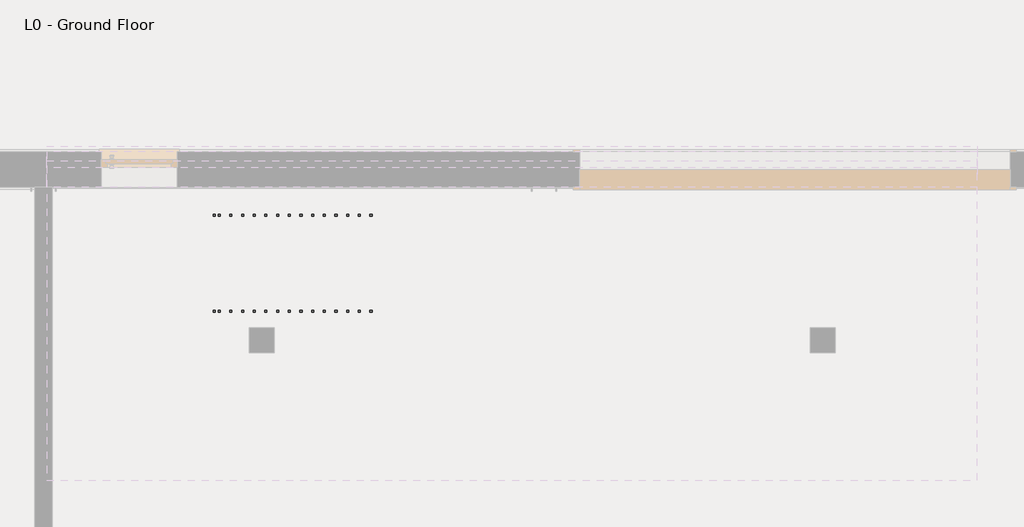
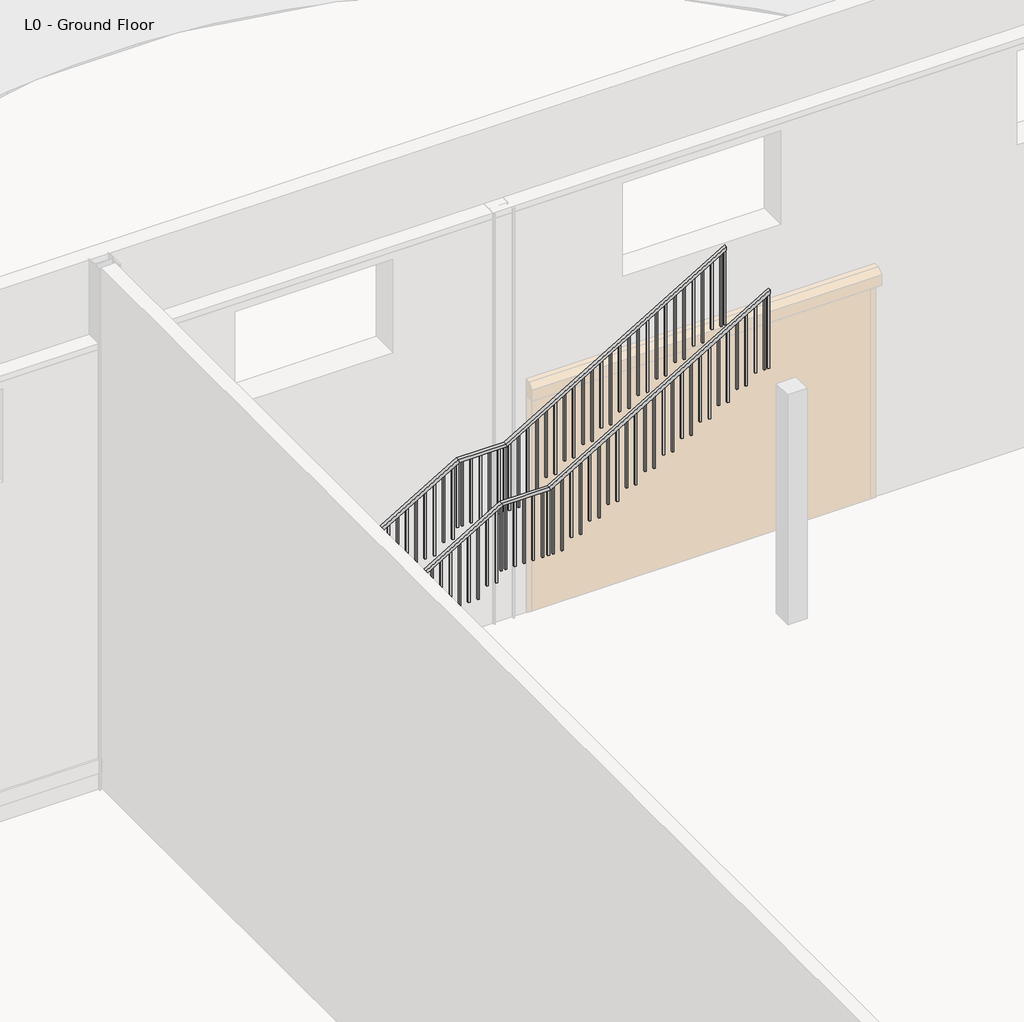
# One storey, part 12 of 14: 2 railings.
"""IFC4 building model written with IfcOpenShell, lengths in millimetres."""

from ifc_helpers import new_model, si_unit, frame, origin, place, context, project, spatial, polyline, outline, extrude, faceted_brep, element, save

model = new_model("IFC4")

# Units and contexts
model_context = context("Model", 3, world=origin())
ifc_project = project(units=[si_unit("LENGTHUNIT", "METRE", prefix="MILLI")], contexts=[model_context])

# Site, building, storey
site = spatial("IfcSite", under=ifc_project)
building = spatial("IfcBuilding", under=site)
storey = spatial("IfcBuildingStorey", under=building, Name="L0 - Ground Floor", Elevation=0.0)

# Railings
placement = place(None, origin())
element("IfcRailing", 1, ObjectType="1100mm", at=placement, inside=storey, context=model_context, shape_type="SolidModel", body=[
    faceted_brep([(12896.9831159, 5374.1380918, 1266.6666667), (12896.9831159, 5374.1380918, 1208.4792885), (12896.9831159, 5324.1380918, 1208.4792885), (12896.9831159, 5324.1380918, 1266.6666667), (15976.9831159, 5374.1380918, 3100.0), (15990.7379111, 5374.1380918, 3050.0), (15990.7379111, 5324.1380918, 3050.0), (15976.9831159, 5324.1380918, 3100.0), (16696.9831159, 5374.1380918, 3100.0), (16710.7379111, 5374.1380918, 3050.0), (16710.7379111, 5324.1380918, 3050.0), (16696.9831159, 5324.1380918, 3100.0), (20056.9831159, 5374.1380918, 5100.0), (20056.9831159, 5324.1380918, 5100.0), (20056.9831159, 5324.1380918, 5041.8126219), (20056.9831159, 5374.1380918, 5041.8126219)], [[[0, 1, 2, 3]], [[1, 0, 4, 5]], [[2, 1, 5, 6]], [[3, 2, 6, 7]], [[0, 3, 7, 4]], [[5, 4, 8, 9]], [[6, 5, 9, 10]], [[7, 6, 10, 11]], [[4, 7, 11, 8]], [[12, 13, 14, 15]], [[9, 8, 12, 15]], [[10, 9, 15, 14]], [[11, 10, 14, 13]], [[8, 11, 13, 12]]]),
    extrude(outline(polyline([(4992.705479, 19974.4831159), (3833.3333333, 19974.4831159), (3833.3333333, 19999.4831159), (5007.5864314, 19999.4831159), (4992.705479, 19974.4831159)])), frame((0.0, 5336.6380918, 0.0), z_axis=(0.0, 1.0, 0.0), x_axis=(0.0, 0.0, 1.0)), (0.0, 0.0, 1.0), 25.0),
    extrude(outline(polyline([(4909.3721457, 19834.4831159), (3833.3333333, 19834.4831159), (3833.3333333, 19859.4831159), (4924.253098, 19859.4831159), (4909.3721457, 19834.4831159)])), frame((0.0, 5336.6380918, 0.0), z_axis=(0.0, 1.0, 0.0), x_axis=(0.0, 0.0, 1.0)), (0.0, 0.0, 1.0), 25.0),
    extrude(outline(polyline([(4826.0388123, 19694.4831159), (3666.6666667, 19694.4831159), (3666.6666667, 19719.4831159), (4840.9197647, 19719.4831159), (4826.0388123, 19694.4831159)])), frame((0.0, 5336.6380918, 0.0), z_axis=(0.0, 1.0, 0.0), x_axis=(0.0, 0.0, 1.0)), (0.0, 0.0, 1.0), 25.0),
    extrude(outline(polyline([(4742.705479, 19554.4831159), (3666.6666667, 19554.4831159), (3666.6666667, 19579.4831159), (4757.5864314, 19579.4831159), (4742.705479, 19554.4831159)])), frame((0.0, 5336.6380918, 0.0), z_axis=(0.0, 1.0, 0.0), x_axis=(0.0, 0.0, 1.0)), (0.0, 0.0, 1.0), 25.0),
    extrude(outline(polyline([(4659.3721457, 19414.4831159), (3500.0, 19414.4831159), (3500.0, 19439.4831159), (4674.253098, 19439.4831159), (4659.3721457, 19414.4831159)])), frame((0.0, 5336.6380918, 0.0), z_axis=(0.0, 1.0, 0.0), x_axis=(0.0, 0.0, 1.0)), (0.0, 0.0, 1.0), 25.0),
    extrude(outline(polyline([(4576.0388123, 19274.4831159), (3500.0, 19274.4831159), (3500.0, 19299.4831159), (4590.9197647, 19299.4831159), (4576.0388123, 19274.4831159)])), frame((0.0, 5336.6380918, 0.0), z_axis=(0.0, 1.0, 0.0), x_axis=(0.0, 0.0, 1.0)), (0.0, 0.0, 1.0), 25.0),
    extrude(outline(polyline([(4492.705479, 19134.4831159), (3333.3333333, 19134.4831159), (3333.3333333, 19159.4831159), (4507.5864314, 19159.4831159), (4492.705479, 19134.4831159)])), frame((0.0, 5336.6380918, 0.0), z_axis=(0.0, 1.0, 0.0), x_axis=(0.0, 0.0, 1.0)), (0.0, 0.0, 1.0), 25.0),
    extrude(outline(polyline([(4409.3721457, 18994.4831159), (3333.3333333, 18994.4831159), (3333.3333333, 19019.4831159), (4424.253098, 19019.4831159), (4409.3721457, 18994.4831159)])), frame((0.0, 5336.6380918, 0.0), z_axis=(0.0, 1.0, 0.0), x_axis=(0.0, 0.0, 1.0)), (0.0, 0.0, 1.0), 25.0),
    extrude(outline(polyline([(4326.0388123, 18854.4831159), (3166.6666667, 18854.4831159), (3166.6666667, 18879.4831159), (4340.9197647, 18879.4831159), (4326.0388123, 18854.4831159)])), frame((0.0, 5336.6380918, 0.0), z_axis=(0.0, 1.0, 0.0), x_axis=(0.0, 0.0, 1.0)), (0.0, 0.0, 1.0), 25.0),
    extrude(outline(polyline([(4242.705479, 18714.4831159), (3166.6666667, 18714.4831159), (3166.6666667, 18739.4831159), (4257.5864314, 18739.4831159), (4242.705479, 18714.4831159)])), frame((0.0, 5336.6380918, 0.0), z_axis=(0.0, 1.0, 0.0), x_axis=(0.0, 0.0, 1.0)), (0.0, 0.0, 1.0), 25.0),
    extrude(outline(polyline([(4159.3721457, 18574.4831159), (3000.0, 18574.4831159), (3000.0, 18599.4831159), (4174.253098, 18599.4831159), (4159.3721457, 18574.4831159)])), frame((0.0, 5336.6380918, 0.0), z_axis=(0.0, 1.0, 0.0), x_axis=(0.0, 0.0, 1.0)), (0.0, 0.0, 1.0), 25.0),
    extrude(outline(polyline([(4076.0388123, 18434.4831159), (3000.0, 18434.4831159), (3000.0, 18459.4831159), (4090.9197647, 18459.4831159), (4076.0388123, 18434.4831159)])), frame((0.0, 5336.6380918, 0.0), z_axis=(0.0, 1.0, 0.0), x_axis=(0.0, 0.0, 1.0)), (0.0, 0.0, 1.0), 25.0),
    extrude(outline(polyline([(3992.705479, 18294.4831159), (2833.3333333, 18294.4831159), (2833.3333333, 18319.4831159), (4007.5864314, 18319.4831159), (3992.705479, 18294.4831159)])), frame((0.0, 5336.6380918, 0.0), z_axis=(0.0, 1.0, 0.0), x_axis=(0.0, 0.0, 1.0)), (0.0, 0.0, 1.0), 25.0),
    extrude(outline(polyline([(3909.3721457, 18154.4831159), (2833.3333333, 18154.4831159), (2833.3333333, 18179.4831159), (3924.253098, 18179.4831159), (3909.3721457, 18154.4831159)])), frame((0.0, 5336.6380918, 0.0), z_axis=(0.0, 1.0, 0.0), x_axis=(0.0, 0.0, 1.0)), (0.0, 0.0, 1.0), 25.0),
    extrude(outline(polyline([(3826.0388123, 18014.4831159), (2666.6666667, 18014.4831159), (2666.6666667, 18039.4831159), (3840.9197647, 18039.4831159), (3826.0388123, 18014.4831159)])), frame((0.0, 5336.6380918, 0.0), z_axis=(0.0, 1.0, 0.0), x_axis=(0.0, 0.0, 1.0)), (0.0, 0.0, 1.0), 25.0),
    extrude(outline(polyline([(3742.705479, 17874.4831159), (2666.6666667, 17874.4831159), (2666.6666667, 17899.4831159), (3757.5864314, 17899.4831159), (3742.705479, 17874.4831159)])), frame((0.0, 5336.6380918, 0.0), z_axis=(0.0, 1.0, 0.0), x_axis=(0.0, 0.0, 1.0)), (0.0, 0.0, 1.0), 25.0),
    extrude(outline(polyline([(3659.3721457, 17734.4831159), (2500.0, 17734.4831159), (2500.0, 17759.4831159), (3674.253098, 17759.4831159), (3659.3721457, 17734.4831159)])), frame((0.0, 5336.6380918, 0.0), z_axis=(0.0, 1.0, 0.0), x_axis=(0.0, 0.0, 1.0)), (0.0, 0.0, 1.0), 25.0),
    extrude(outline(polyline([(3576.0388123, 17594.4831159), (2500.0, 17594.4831159), (2500.0, 17619.4831159), (3590.9197647, 17619.4831159), (3576.0388123, 17594.4831159)])), frame((0.0, 5336.6380918, 0.0), z_axis=(0.0, 1.0, 0.0), x_axis=(0.0, 0.0, 1.0)), (0.0, 0.0, 1.0), 25.0),
    extrude(outline(polyline([(3492.705479, 17454.4831159), (2333.3333333, 17454.4831159), (2333.3333333, 17479.4831159), (3507.5864314, 17479.4831159), (3492.705479, 17454.4831159)])), frame((0.0, 5336.6380918, 0.0), z_axis=(0.0, 1.0, 0.0), x_axis=(0.0, 0.0, 1.0)), (0.0, 0.0, 1.0), 25.0),
    extrude(outline(polyline([(3409.3721457, 17314.4831159), (2333.3333333, 17314.4831159), (2333.3333333, 17339.4831159), (3424.253098, 17339.4831159), (3409.3721457, 17314.4831159)])), frame((0.0, 5336.6380918, 0.0), z_axis=(0.0, 1.0, 0.0), x_axis=(0.0, 0.0, 1.0)), (0.0, 0.0, 1.0), 25.0),
    extrude(outline(polyline([(3326.0388123, 17174.4831159), (2166.6666667, 17174.4831159), (2166.6666667, 17199.4831159), (3340.9197647, 17199.4831159), (3326.0388123, 17174.4831159)])), frame((0.0, 5336.6380918, 0.0), z_axis=(0.0, 1.0, 0.0), x_axis=(0.0, 0.0, 1.0)), (0.0, 0.0, 1.0), 25.0),
    extrude(outline(polyline([(3242.705479, 17034.4831159), (2166.6666667, 17034.4831159), (2166.6666667, 17059.4831159), (3257.5864314, 17059.4831159), (3242.705479, 17034.4831159)])), frame((0.0, 5336.6380918, 0.0), z_axis=(0.0, 1.0, 0.0), x_axis=(0.0, 0.0, 1.0)), (0.0, 0.0, 1.0), 25.0),
    extrude(outline(polyline([(3159.3721457, 16894.4831159), (2000.0, 16894.4831159), (2000.0, 16919.4831159), (3174.253098, 16919.4831159), (3159.3721457, 16894.4831159)])), frame((0.0, 5336.6380918, 0.0), z_axis=(0.0, 1.0, 0.0), x_axis=(0.0, 0.0, 1.0)), (0.0, 0.0, 1.0), 25.0),
    extrude(outline(polyline([(3076.0388123, 16754.4831159), (2000.0, 16754.4831159), (2000.0, 16779.4831159), (3090.9197647, 16779.4831159), (3076.0388123, 16754.4831159)])), frame((0.0, 5336.6380918, 0.0), z_axis=(0.0, 1.0, 0.0), x_axis=(0.0, 0.0, 1.0)), (0.0, 0.0, 1.0), 25.0),
    extrude(outline(polyline([(16594.4831159, 5336.6380918), (16594.4831159, 5361.6380918), (16619.4831159, 5361.6380918), (16619.4831159, 5336.6380918), (16594.4831159, 5336.6380918)])), frame((0.0, 0.0, 2000.0), z_axis=(0.0, 0.0, 1.0), x_axis=(1.0, 0.0, 0.0)), (0.0, 0.0, 1.0), 1050.0),
    extrude(outline(polyline([(16454.4831159, 5336.6380918), (16454.4831159, 5361.6380918), (16479.4831159, 5361.6380918), (16479.4831159, 5336.6380918), (16454.4831159, 5336.6380918)])), frame((0.0, 0.0, 2000.0), z_axis=(0.0, 0.0, 1.0), x_axis=(1.0, 0.0, 0.0)), (0.0, 0.0, 1.0), 1050.0),
    extrude(outline(polyline([(16314.4831159, 5336.6380918), (16314.4831159, 5361.6380918), (16339.4831159, 5361.6380918), (16339.4831159, 5336.6380918), (16314.4831159, 5336.6380918)])), frame((0.0, 0.0, 2000.0), z_axis=(0.0, 0.0, 1.0), x_axis=(1.0, 0.0, 0.0)), (0.0, 0.0, 1.0), 1050.0),
    extrude(outline(polyline([(16174.4831159, 5336.6380918), (16174.4831159, 5361.6380918), (16199.4831159, 5361.6380918), (16199.4831159, 5336.6380918), (16174.4831159, 5336.6380918)])), frame((0.0, 0.0, 2000.0), z_axis=(0.0, 0.0, 1.0), x_axis=(1.0, 0.0, 0.0)), (0.0, 0.0, 1.0), 1050.0),
    extrude(outline(polyline([(16034.4831159, 5336.6380918), (16034.4831159, 5361.6380918), (16059.4831159, 5361.6380918), (16059.4831159, 5336.6380918), (16034.4831159, 5336.6380918)])), frame((0.0, 0.0, 2000.0), z_axis=(0.0, 0.0, 1.0), x_axis=(1.0, 0.0, 0.0)), (0.0, 0.0, 1.0), 1050.0),
    extrude(outline(polyline([(2992.705479, 15894.4831159), (1833.3333333, 15894.4831159), (1833.3333333, 15919.4831159), (3007.5864314, 15919.4831159), (2992.705479, 15894.4831159)])), frame((0.0, 5336.6380918, 0.0), z_axis=(0.0, 1.0, 0.0), x_axis=(0.0, 0.0, 1.0)), (0.0, 0.0, 1.0), 25.0),
    extrude(outline(polyline([(2909.3721457, 15754.4831159), (1833.3333333, 15754.4831159), (1833.3333333, 15779.4831159), (2924.253098, 15779.4831159), (2909.3721457, 15754.4831159)])), frame((0.0, 5336.6380918, 0.0), z_axis=(0.0, 1.0, 0.0), x_axis=(0.0, 0.0, 1.0)), (0.0, 0.0, 1.0), 25.0),
    extrude(outline(polyline([(2826.0388123, 15614.4831159), (1666.6666667, 15614.4831159), (1666.6666667, 15639.4831159), (2840.9197647, 15639.4831159), (2826.0388123, 15614.4831159)])), frame((0.0, 5336.6380918, 0.0), z_axis=(0.0, 1.0, 0.0), x_axis=(0.0, 0.0, 1.0)), (0.0, 0.0, 1.0), 25.0),
    extrude(outline(polyline([(2742.705479, 15474.4831159), (1666.6666667, 15474.4831159), (1666.6666667, 15499.4831159), (2757.5864314, 15499.4831159), (2742.705479, 15474.4831159)])), frame((0.0, 5336.6380918, 0.0), z_axis=(0.0, 1.0, 0.0), x_axis=(0.0, 0.0, 1.0)), (0.0, 0.0, 1.0), 25.0),
    extrude(outline(polyline([(2659.3721457, 15334.4831159), (1500.0, 15334.4831159), (1500.0, 15359.4831159), (2674.253098, 15359.4831159), (2659.3721457, 15334.4831159)])), frame((0.0, 5336.6380918, 0.0), z_axis=(0.0, 1.0, 0.0), x_axis=(0.0, 0.0, 1.0)), (0.0, 0.0, 1.0), 25.0),
    extrude(outline(polyline([(2576.0388123, 15194.4831159), (1500.0, 15194.4831159), (1500.0, 15219.4831159), (2590.9197647, 15219.4831159), (2576.0388123, 15194.4831159)])), frame((0.0, 5336.6380918, 0.0), z_axis=(0.0, 1.0, 0.0), x_axis=(0.0, 0.0, 1.0)), (0.0, 0.0, 1.0), 25.0),
    extrude(outline(polyline([(2492.705479, 15054.4831159), (1333.3333333, 15054.4831159), (1333.3333333, 15079.4831159), (2507.5864314, 15079.4831159), (2492.705479, 15054.4831159)])), frame((0.0, 5336.6380918, 0.0), z_axis=(0.0, 1.0, 0.0), x_axis=(0.0, 0.0, 1.0)), (0.0, 0.0, 1.0), 25.0),
    extrude(outline(polyline([(2409.3721457, 14914.4831159), (1333.3333333, 14914.4831159), (1333.3333333, 14939.4831159), (2424.253098, 14939.4831159), (2409.3721457, 14914.4831159)])), frame((0.0, 5336.6380918, 0.0), z_axis=(0.0, 1.0, 0.0), x_axis=(0.0, 0.0, 1.0)), (0.0, 0.0, 1.0), 25.0),
    extrude(outline(polyline([(2326.0388123, 14774.4831159), (1166.6666667, 14774.4831159), (1166.6666667, 14799.4831159), (2340.9197647, 14799.4831159), (2326.0388123, 14774.4831159)])), frame((0.0, 5336.6380918, 0.0), z_axis=(0.0, 1.0, 0.0), x_axis=(0.0, 0.0, 1.0)), (0.0, 0.0, 1.0), 25.0),
    extrude(outline(polyline([(2242.705479, 14634.4831159), (1166.6666667, 14634.4831159), (1166.6666667, 14659.4831159), (2257.5864314, 14659.4831159), (2242.705479, 14634.4831159)])), frame((0.0, 5336.6380918, 0.0), z_axis=(0.0, 1.0, 0.0), x_axis=(0.0, 0.0, 1.0)), (0.0, 0.0, 1.0), 25.0),
    extrude(outline(polyline([(2159.3721457, 14494.4831159), (1000.0, 14494.4831159), (1000.0, 14519.4831159), (2174.253098, 14519.4831159), (2159.3721457, 14494.4831159)])), frame((0.0, 5336.6380918, 0.0), z_axis=(0.0, 1.0, 0.0), x_axis=(0.0, 0.0, 1.0)), (0.0, 0.0, 1.0), 25.0),
    extrude(outline(polyline([(2076.0388123, 14354.4831159), (1000.0, 14354.4831159), (1000.0, 14379.4831159), (2090.9197647, 14379.4831159), (2076.0388123, 14354.4831159)])), frame((0.0, 5336.6380918, 0.0), z_axis=(0.0, 1.0, 0.0), x_axis=(0.0, 0.0, 1.0)), (0.0, 0.0, 1.0), 25.0),
    extrude(outline(polyline([(1992.705479, 14214.4831159), (833.3333333, 14214.4831159), (833.3333333, 14239.4831159), (2007.5864314, 14239.4831159), (1992.705479, 14214.4831159)])), frame((0.0, 5336.6380918, 0.0), z_axis=(0.0, 1.0, 0.0), x_axis=(0.0, 0.0, 1.0)), (0.0, 0.0, 1.0), 25.0),
    extrude(outline(polyline([(1909.3721457, 14074.4831159), (833.3333333, 14074.4831159), (833.3333333, 14099.4831159), (1924.253098, 14099.4831159), (1909.3721457, 14074.4831159)])), frame((0.0, 5336.6380918, 0.0), z_axis=(0.0, 1.0, 0.0), x_axis=(0.0, 0.0, 1.0)), (0.0, 0.0, 1.0), 25.0),
    extrude(outline(polyline([(1826.0388123, 13934.4831159), (666.6666667, 13934.4831159), (666.6666667, 13959.4831159), (1840.9197647, 13959.4831159), (1826.0388123, 13934.4831159)])), frame((0.0, 5336.6380918, 0.0), z_axis=(0.0, 1.0, 0.0), x_axis=(0.0, 0.0, 1.0)), (0.0, 0.0, 1.0), 25.0),
    extrude(outline(polyline([(1742.705479, 13794.4831159), (666.6666667, 13794.4831159), (666.6666667, 13819.4831159), (1757.5864314, 13819.4831159), (1742.705479, 13794.4831159)])), frame((0.0, 5336.6380918, 0.0), z_axis=(0.0, 1.0, 0.0), x_axis=(0.0, 0.0, 1.0)), (0.0, 0.0, 1.0), 25.0),
    extrude(outline(polyline([(1659.3721457, 13654.4831159), (500.0, 13654.4831159), (500.0, 13679.4831159), (1674.253098, 13679.4831159), (1659.3721457, 13654.4831159)])), frame((0.0, 5336.6380918, 0.0), z_axis=(0.0, 1.0, 0.0), x_axis=(0.0, 0.0, 1.0)), (0.0, 0.0, 1.0), 25.0),
    extrude(outline(polyline([(1576.0388123, 13514.4831159), (500.0, 13514.4831159), (500.0, 13539.4831159), (1590.9197647, 13539.4831159), (1576.0388123, 13514.4831159)])), frame((0.0, 5336.6380918, 0.0), z_axis=(0.0, 1.0, 0.0), x_axis=(0.0, 0.0, 1.0)), (0.0, 0.0, 1.0), 25.0),
    extrude(outline(polyline([(1492.705479, 13374.4831159), (333.3333333, 13374.4831159), (333.3333333, 13399.4831159), (1507.5864314, 13399.4831159), (1492.705479, 13374.4831159)])), frame((0.0, 5336.6380918, 0.0), z_axis=(0.0, 1.0, 0.0), x_axis=(0.0, 0.0, 1.0)), (0.0, 0.0, 1.0), 25.0),
    extrude(outline(polyline([(1409.3721457, 13234.4831159), (333.3333333, 13234.4831159), (333.3333333, 13259.4831159), (1424.253098, 13259.4831159), (1409.3721457, 13234.4831159)])), frame((0.0, 5336.6380918, 0.0), z_axis=(0.0, 1.0, 0.0), x_axis=(0.0, 0.0, 1.0)), (0.0, 0.0, 1.0), 25.0),
    extrude(outline(polyline([(1326.0388123, 13094.4831159), (166.6666667, 13094.4831159), (166.6666667, 13119.4831159), (1340.9197647, 13119.4831159), (1326.0388123, 13094.4831159)])), frame((0.0, 5336.6380918, 0.0), z_axis=(0.0, 1.0, 0.0), x_axis=(0.0, 0.0, 1.0)), (0.0, 0.0, 1.0), 25.0),
    extrude(outline(polyline([(1242.705479, 12954.4831159), (166.6666667, 12954.4831159), (166.6666667, 12979.4831159), (1257.5864314, 12979.4831159), (1242.705479, 12954.4831159)])), frame((0.0, 5336.6380918, 0.0), z_axis=(0.0, 1.0, 0.0), x_axis=(0.0, 0.0, 1.0)), (0.0, 0.0, 1.0), 25.0),
    extrude(outline(polyline([(16684.4831159, 5336.6380918), (16684.4831159, 5361.6380918), (16709.4831159, 5361.6380918), (16709.4831159, 5336.6380918), (16684.4831159, 5336.6380918)])), frame((0.0, 0.0, 2000.0), z_axis=(0.0, 0.0, 1.0), x_axis=(1.0, 0.0, 0.0)), (0.0, 0.0, 1.0), 1050.0),
    extrude(outline(polyline([(15964.4831159, 5336.6380918), (15964.4831159, 5361.6380918), (15989.4831159, 5361.6380918), (15989.4831159, 5336.6380918), (15964.4831159, 5336.6380918)])), frame((0.0, 0.0, 2000.0), z_axis=(0.0, 0.0, 1.0), x_axis=(1.0, 0.0, 0.0)), (0.0, 0.0, 1.0), 1050.0),
    extrude(outline(polyline([(5026.9316695, 20031.9831159), (3833.3333333, 20031.9831159), (3833.3333333, 20056.9831159), (5041.8126219, 20056.9831159), (5026.9316695, 20031.9831159)])), frame((0.0, 5336.6380918, 0.0), z_axis=(0.0, 1.0, 0.0), x_axis=(0.0, 0.0, 1.0)), (0.0, 0.0, 1.0), 25.0),
    extrude(outline(polyline([(1208.4792885, 12896.9831159), (166.6666667, 12896.9831159), (166.6666667, 12921.9831159), (1223.3602409, 12921.9831159), (1208.4792885, 12896.9831159)])), frame((0.0, 5336.6380918, 0.0), z_axis=(0.0, 1.0, 0.0), x_axis=(0.0, 0.0, 1.0)), (0.0, 0.0, 1.0), 25.0),
])
element("IfcRailing", 2, ObjectType="1100mm", at=placement, inside=storey, context=model_context, shape_type="SolidModel", body=[
    faceted_brep([(12896.9831159, 6523.3380918, 1266.6666667), (12896.9831159, 6523.3380918, 1208.4792885), (12896.9831159, 6473.3380918, 1208.4792885), (12896.9831159, 6473.3380918, 1266.6666667), (15976.9831159, 6523.3380918, 3100.0), (15990.7379111, 6523.3380918, 3050.0), (15990.7379111, 6473.3380918, 3050.0), (15976.9831159, 6473.3380918, 3100.0), (16696.9831159, 6523.3380918, 3100.0), (16710.7379111, 6523.3380918, 3050.0), (16710.7379111, 6473.3380918, 3050.0), (16696.9831159, 6473.3380918, 3100.0), (20056.9831159, 6523.3380918, 5100.0), (20056.9831159, 6473.3380918, 5100.0), (20056.9831159, 6473.3380918, 5041.8126219), (20056.9831159, 6523.3380918, 5041.8126219)], [[[0, 1, 2, 3]], [[1, 0, 4, 5]], [[2, 1, 5, 6]], [[3, 2, 6, 7]], [[0, 3, 7, 4]], [[5, 4, 8, 9]], [[6, 5, 9, 10]], [[7, 6, 10, 11]], [[4, 7, 11, 8]], [[12, 13, 14, 15]], [[9, 8, 12, 15]], [[10, 9, 15, 14]], [[11, 10, 14, 13]], [[8, 11, 13, 12]]]),
    extrude(outline(polyline([(3833.3333333, 19974.4831159), (3833.3333333, 19999.4831159), (5007.5864314, 19999.4831159), (4992.705479, 19974.4831159), (3833.3333333, 19974.4831159)])), frame((0.0, 6485.8380918, 0.0), z_axis=(0.0, 1.0, 0.0), x_axis=(0.0, 0.0, 1.0)), (0.0, 0.0, 1.0), 25.0),
    extrude(outline(polyline([(3833.3333333, 19834.4831159), (3833.3333333, 19859.4831159), (4924.253098, 19859.4831159), (4909.3721457, 19834.4831159), (3833.3333333, 19834.4831159)])), frame((0.0, 6485.8380918, 0.0), z_axis=(0.0, 1.0, 0.0), x_axis=(0.0, 0.0, 1.0)), (0.0, 0.0, 1.0), 25.0),
    extrude(outline(polyline([(3666.6666667, 19694.4831159), (3666.6666667, 19719.4831159), (4840.9197647, 19719.4831159), (4826.0388123, 19694.4831159), (3666.6666667, 19694.4831159)])), frame((0.0, 6485.8380918, 0.0), z_axis=(0.0, 1.0, 0.0), x_axis=(0.0, 0.0, 1.0)), (0.0, 0.0, 1.0), 25.0),
    extrude(outline(polyline([(3666.6666667, 19554.4831159), (3666.6666667, 19579.4831159), (4757.5864314, 19579.4831159), (4742.705479, 19554.4831159), (3666.6666667, 19554.4831159)])), frame((0.0, 6485.8380918, 0.0), z_axis=(0.0, 1.0, 0.0), x_axis=(0.0, 0.0, 1.0)), (0.0, 0.0, 1.0), 25.0),
    extrude(outline(polyline([(3500.0, 19414.4831159), (3500.0, 19439.4831159), (4674.253098, 19439.4831159), (4659.3721457, 19414.4831159), (3500.0, 19414.4831159)])), frame((0.0, 6485.8380918, 0.0), z_axis=(0.0, 1.0, 0.0), x_axis=(0.0, 0.0, 1.0)), (0.0, 0.0, 1.0), 25.0),
    extrude(outline(polyline([(3500.0, 19274.4831159), (3500.0, 19299.4831159), (4590.9197647, 19299.4831159), (4576.0388123, 19274.4831159), (3500.0, 19274.4831159)])), frame((0.0, 6485.8380918, 0.0), z_axis=(0.0, 1.0, 0.0), x_axis=(0.0, 0.0, 1.0)), (0.0, 0.0, 1.0), 25.0),
    extrude(outline(polyline([(3333.3333333, 19134.4831159), (3333.3333333, 19159.4831159), (4507.5864314, 19159.4831159), (4492.705479, 19134.4831159), (3333.3333333, 19134.4831159)])), frame((0.0, 6485.8380918, 0.0), z_axis=(0.0, 1.0, 0.0), x_axis=(0.0, 0.0, 1.0)), (0.0, 0.0, 1.0), 25.0),
    extrude(outline(polyline([(3333.3333333, 18994.4831159), (3333.3333333, 19019.4831159), (4424.253098, 19019.4831159), (4409.3721457, 18994.4831159), (3333.3333333, 18994.4831159)])), frame((0.0, 6485.8380918, 0.0), z_axis=(0.0, 1.0, 0.0), x_axis=(0.0, 0.0, 1.0)), (0.0, 0.0, 1.0), 25.0),
    extrude(outline(polyline([(3166.6666667, 18854.4831159), (3166.6666667, 18879.4831159), (4340.9197647, 18879.4831159), (4326.0388123, 18854.4831159), (3166.6666667, 18854.4831159)])), frame((0.0, 6485.8380918, 0.0), z_axis=(0.0, 1.0, 0.0), x_axis=(0.0, 0.0, 1.0)), (0.0, 0.0, 1.0), 25.0),
    extrude(outline(polyline([(3166.6666667, 18714.4831159), (3166.6666667, 18739.4831159), (4257.5864314, 18739.4831159), (4242.705479, 18714.4831159), (3166.6666667, 18714.4831159)])), frame((0.0, 6485.8380918, 0.0), z_axis=(0.0, 1.0, 0.0), x_axis=(0.0, 0.0, 1.0)), (0.0, 0.0, 1.0), 25.0),
    extrude(outline(polyline([(3000.0, 18574.4831159), (3000.0, 18599.4831159), (4174.253098, 18599.4831159), (4159.3721457, 18574.4831159), (3000.0, 18574.4831159)])), frame((0.0, 6485.8380918, 0.0), z_axis=(0.0, 1.0, 0.0), x_axis=(0.0, 0.0, 1.0)), (0.0, 0.0, 1.0), 25.0),
    extrude(outline(polyline([(3000.0, 18434.4831159), (3000.0, 18459.4831159), (4090.9197647, 18459.4831159), (4076.0388123, 18434.4831159), (3000.0, 18434.4831159)])), frame((0.0, 6485.8380918, 0.0), z_axis=(0.0, 1.0, 0.0), x_axis=(0.0, 0.0, 1.0)), (0.0, 0.0, 1.0), 25.0),
    extrude(outline(polyline([(2833.3333333, 18294.4831159), (2833.3333333, 18319.4831159), (4007.5864314, 18319.4831159), (3992.705479, 18294.4831159), (2833.3333333, 18294.4831159)])), frame((0.0, 6485.8380918, 0.0), z_axis=(0.0, 1.0, 0.0), x_axis=(0.0, 0.0, 1.0)), (0.0, 0.0, 1.0), 25.0),
    extrude(outline(polyline([(2833.3333333, 18154.4831159), (2833.3333333, 18179.4831159), (3924.253098, 18179.4831159), (3909.3721457, 18154.4831159), (2833.3333333, 18154.4831159)])), frame((0.0, 6485.8380918, 0.0), z_axis=(0.0, 1.0, 0.0), x_axis=(0.0, 0.0, 1.0)), (0.0, 0.0, 1.0), 25.0),
    extrude(outline(polyline([(2666.6666667, 18014.4831159), (2666.6666667, 18039.4831159), (3840.9197647, 18039.4831159), (3826.0388123, 18014.4831159), (2666.6666667, 18014.4831159)])), frame((0.0, 6485.8380918, 0.0), z_axis=(0.0, 1.0, 0.0), x_axis=(0.0, 0.0, 1.0)), (0.0, 0.0, 1.0), 25.0),
    extrude(outline(polyline([(2666.6666667, 17874.4831159), (2666.6666667, 17899.4831159), (3757.5864314, 17899.4831159), (3742.705479, 17874.4831159), (2666.6666667, 17874.4831159)])), frame((0.0, 6485.8380918, 0.0), z_axis=(0.0, 1.0, 0.0), x_axis=(0.0, 0.0, 1.0)), (0.0, 0.0, 1.0), 25.0),
    extrude(outline(polyline([(2500.0, 17734.4831159), (2500.0, 17759.4831159), (3674.253098, 17759.4831159), (3659.3721457, 17734.4831159), (2500.0, 17734.4831159)])), frame((0.0, 6485.8380918, 0.0), z_axis=(0.0, 1.0, 0.0), x_axis=(0.0, 0.0, 1.0)), (0.0, 0.0, 1.0), 25.0),
    extrude(outline(polyline([(2500.0, 17594.4831159), (2500.0, 17619.4831159), (3590.9197647, 17619.4831159), (3576.0388123, 17594.4831159), (2500.0, 17594.4831159)])), frame((0.0, 6485.8380918, 0.0), z_axis=(0.0, 1.0, 0.0), x_axis=(0.0, 0.0, 1.0)), (0.0, 0.0, 1.0), 25.0),
    extrude(outline(polyline([(2333.3333333, 17454.4831159), (2333.3333333, 17479.4831159), (3507.5864314, 17479.4831159), (3492.705479, 17454.4831159), (2333.3333333, 17454.4831159)])), frame((0.0, 6485.8380918, 0.0), z_axis=(0.0, 1.0, 0.0), x_axis=(0.0, 0.0, 1.0)), (0.0, 0.0, 1.0), 25.0),
    extrude(outline(polyline([(2333.3333333, 17314.4831159), (2333.3333333, 17339.4831159), (3424.253098, 17339.4831159), (3409.3721457, 17314.4831159), (2333.3333333, 17314.4831159)])), frame((0.0, 6485.8380918, 0.0), z_axis=(0.0, 1.0, 0.0), x_axis=(0.0, 0.0, 1.0)), (0.0, 0.0, 1.0), 25.0),
    extrude(outline(polyline([(2166.6666667, 17174.4831159), (2166.6666667, 17199.4831159), (3340.9197647, 17199.4831159), (3326.0388123, 17174.4831159), (2166.6666667, 17174.4831159)])), frame((0.0, 6485.8380918, 0.0), z_axis=(0.0, 1.0, 0.0), x_axis=(0.0, 0.0, 1.0)), (0.0, 0.0, 1.0), 25.0),
    extrude(outline(polyline([(2166.6666667, 17034.4831159), (2166.6666667, 17059.4831159), (3257.5864314, 17059.4831159), (3242.705479, 17034.4831159), (2166.6666667, 17034.4831159)])), frame((0.0, 6485.8380918, 0.0), z_axis=(0.0, 1.0, 0.0), x_axis=(0.0, 0.0, 1.0)), (0.0, 0.0, 1.0), 25.0),
    extrude(outline(polyline([(2000.0, 16894.4831159), (2000.0, 16919.4831159), (3174.253098, 16919.4831159), (3159.3721457, 16894.4831159), (2000.0, 16894.4831159)])), frame((0.0, 6485.8380918, 0.0), z_axis=(0.0, 1.0, 0.0), x_axis=(0.0, 0.0, 1.0)), (0.0, 0.0, 1.0), 25.0),
    extrude(outline(polyline([(2000.0, 16754.4831159), (2000.0, 16779.4831159), (3090.9197647, 16779.4831159), (3076.0388123, 16754.4831159), (2000.0, 16754.4831159)])), frame((0.0, 6485.8380918, 0.0), z_axis=(0.0, 1.0, 0.0), x_axis=(0.0, 0.0, 1.0)), (0.0, 0.0, 1.0), 25.0),
    extrude(outline(polyline([(16594.4831159, 6510.8380918), (16619.4831159, 6510.8380918), (16619.4831159, 6485.8380918), (16594.4831159, 6485.8380918), (16594.4831159, 6510.8380918)])), frame((0.0, 0.0, 2000.0), z_axis=(0.0, 0.0, 1.0), x_axis=(1.0, 0.0, 0.0)), (0.0, 0.0, 1.0), 1050.0),
    extrude(outline(polyline([(16454.4831159, 6510.8380918), (16479.4831159, 6510.8380918), (16479.4831159, 6485.8380918), (16454.4831159, 6485.8380918), (16454.4831159, 6510.8380918)])), frame((0.0, 0.0, 2000.0), z_axis=(0.0, 0.0, 1.0), x_axis=(1.0, 0.0, 0.0)), (0.0, 0.0, 1.0), 1050.0),
    extrude(outline(polyline([(16314.4831159, 6510.8380918), (16339.4831159, 6510.8380918), (16339.4831159, 6485.8380918), (16314.4831159, 6485.8380918), (16314.4831159, 6510.8380918)])), frame((0.0, 0.0, 2000.0), z_axis=(0.0, 0.0, 1.0), x_axis=(1.0, 0.0, 0.0)), (0.0, 0.0, 1.0), 1050.0),
    extrude(outline(polyline([(16174.4831159, 6510.8380918), (16199.4831159, 6510.8380918), (16199.4831159, 6485.8380918), (16174.4831159, 6485.8380918), (16174.4831159, 6510.8380918)])), frame((0.0, 0.0, 2000.0), z_axis=(0.0, 0.0, 1.0), x_axis=(1.0, 0.0, 0.0)), (0.0, 0.0, 1.0), 1050.0),
    extrude(outline(polyline([(16034.4831159, 6510.8380918), (16059.4831159, 6510.8380918), (16059.4831159, 6485.8380918), (16034.4831159, 6485.8380918), (16034.4831159, 6510.8380918)])), frame((0.0, 0.0, 2000.0), z_axis=(0.0, 0.0, 1.0), x_axis=(1.0, 0.0, 0.0)), (0.0, 0.0, 1.0), 1050.0),
    extrude(outline(polyline([(1833.3333333, 15894.4831159), (1833.3333333, 15919.4831159), (3007.5864314, 15919.4831159), (2992.705479, 15894.4831159), (1833.3333333, 15894.4831159)])), frame((0.0, 6485.8380918, 0.0), z_axis=(0.0, 1.0, 0.0), x_axis=(0.0, 0.0, 1.0)), (0.0, 0.0, 1.0), 25.0),
    extrude(outline(polyline([(1833.3333333, 15754.4831159), (1833.3333333, 15779.4831159), (2924.253098, 15779.4831159), (2909.3721457, 15754.4831159), (1833.3333333, 15754.4831159)])), frame((0.0, 6485.8380918, 0.0), z_axis=(0.0, 1.0, 0.0), x_axis=(0.0, 0.0, 1.0)), (0.0, 0.0, 1.0), 25.0),
    extrude(outline(polyline([(1666.6666667, 15614.4831159), (1666.6666667, 15639.4831159), (2840.9197647, 15639.4831159), (2826.0388123, 15614.4831159), (1666.6666667, 15614.4831159)])), frame((0.0, 6485.8380918, 0.0), z_axis=(0.0, 1.0, 0.0), x_axis=(0.0, 0.0, 1.0)), (0.0, 0.0, 1.0), 25.0),
    extrude(outline(polyline([(1666.6666667, 15474.4831159), (1666.6666667, 15499.4831159), (2757.5864314, 15499.4831159), (2742.705479, 15474.4831159), (1666.6666667, 15474.4831159)])), frame((0.0, 6485.8380918, 0.0), z_axis=(0.0, 1.0, 0.0), x_axis=(0.0, 0.0, 1.0)), (0.0, 0.0, 1.0), 25.0),
    extrude(outline(polyline([(1500.0, 15334.4831159), (1500.0, 15359.4831159), (2674.253098, 15359.4831159), (2659.3721457, 15334.4831159), (1500.0, 15334.4831159)])), frame((0.0, 6485.8380918, 0.0), z_axis=(0.0, 1.0, 0.0), x_axis=(0.0, 0.0, 1.0)), (0.0, 0.0, 1.0), 25.0),
    extrude(outline(polyline([(1500.0, 15194.4831159), (1500.0, 15219.4831159), (2590.9197647, 15219.4831159), (2576.0388123, 15194.4831159), (1500.0, 15194.4831159)])), frame((0.0, 6485.8380918, 0.0), z_axis=(0.0, 1.0, 0.0), x_axis=(0.0, 0.0, 1.0)), (0.0, 0.0, 1.0), 25.0),
    extrude(outline(polyline([(1333.3333333, 15054.4831159), (1333.3333333, 15079.4831159), (2507.5864314, 15079.4831159), (2492.705479, 15054.4831159), (1333.3333333, 15054.4831159)])), frame((0.0, 6485.8380918, 0.0), z_axis=(0.0, 1.0, 0.0), x_axis=(0.0, 0.0, 1.0)), (0.0, 0.0, 1.0), 25.0),
    extrude(outline(polyline([(1333.3333333, 14914.4831159), (1333.3333333, 14939.4831159), (2424.253098, 14939.4831159), (2409.3721457, 14914.4831159), (1333.3333333, 14914.4831159)])), frame((0.0, 6485.8380918, 0.0), z_axis=(0.0, 1.0, 0.0), x_axis=(0.0, 0.0, 1.0)), (0.0, 0.0, 1.0), 25.0),
    extrude(outline(polyline([(1166.6666667, 14774.4831159), (1166.6666667, 14799.4831159), (2340.9197647, 14799.4831159), (2326.0388123, 14774.4831159), (1166.6666667, 14774.4831159)])), frame((0.0, 6485.8380918, 0.0), z_axis=(0.0, 1.0, 0.0), x_axis=(0.0, 0.0, 1.0)), (0.0, 0.0, 1.0), 25.0),
    extrude(outline(polyline([(1166.6666667, 14634.4831159), (1166.6666667, 14659.4831159), (2257.5864314, 14659.4831159), (2242.705479, 14634.4831159), (1166.6666667, 14634.4831159)])), frame((0.0, 6485.8380918, 0.0), z_axis=(0.0, 1.0, 0.0), x_axis=(0.0, 0.0, 1.0)), (0.0, 0.0, 1.0), 25.0),
    extrude(outline(polyline([(1000.0, 14494.4831159), (1000.0, 14519.4831159), (2174.253098, 14519.4831159), (2159.3721457, 14494.4831159), (1000.0, 14494.4831159)])), frame((0.0, 6485.8380918, 0.0), z_axis=(0.0, 1.0, 0.0), x_axis=(0.0, 0.0, 1.0)), (0.0, 0.0, 1.0), 25.0),
    extrude(outline(polyline([(1000.0, 14354.4831159), (1000.0, 14379.4831159), (2090.9197647, 14379.4831159), (2076.0388123, 14354.4831159), (1000.0, 14354.4831159)])), frame((0.0, 6485.8380918, 0.0), z_axis=(0.0, 1.0, 0.0), x_axis=(0.0, 0.0, 1.0)), (0.0, 0.0, 1.0), 25.0),
    extrude(outline(polyline([(833.3333333, 14214.4831159), (833.3333333, 14239.4831159), (2007.5864314, 14239.4831159), (1992.705479, 14214.4831159), (833.3333333, 14214.4831159)])), frame((0.0, 6485.8380918, 0.0), z_axis=(0.0, 1.0, 0.0), x_axis=(0.0, 0.0, 1.0)), (0.0, 0.0, 1.0), 25.0),
    extrude(outline(polyline([(833.3333333, 14074.4831159), (833.3333333, 14099.4831159), (1924.253098, 14099.4831159), (1909.3721457, 14074.4831159), (833.3333333, 14074.4831159)])), frame((0.0, 6485.8380918, 0.0), z_axis=(0.0, 1.0, 0.0), x_axis=(0.0, 0.0, 1.0)), (0.0, 0.0, 1.0), 25.0),
    extrude(outline(polyline([(666.6666667, 13934.4831159), (666.6666667, 13959.4831159), (1840.9197647, 13959.4831159), (1826.0388123, 13934.4831159), (666.6666667, 13934.4831159)])), frame((0.0, 6485.8380918, 0.0), z_axis=(0.0, 1.0, 0.0), x_axis=(0.0, 0.0, 1.0)), (0.0, 0.0, 1.0), 25.0),
    extrude(outline(polyline([(666.6666667, 13794.4831159), (666.6666667, 13819.4831159), (1757.5864314, 13819.4831159), (1742.705479, 13794.4831159), (666.6666667, 13794.4831159)])), frame((0.0, 6485.8380918, 0.0), z_axis=(0.0, 1.0, 0.0), x_axis=(0.0, 0.0, 1.0)), (0.0, 0.0, 1.0), 25.0),
    extrude(outline(polyline([(500.0, 13654.4831159), (500.0, 13679.4831159), (1674.253098, 13679.4831159), (1659.3721457, 13654.4831159), (500.0, 13654.4831159)])), frame((0.0, 6485.8380918, 0.0), z_axis=(0.0, 1.0, 0.0), x_axis=(0.0, 0.0, 1.0)), (0.0, 0.0, 1.0), 25.0),
    extrude(outline(polyline([(500.0, 13514.4831159), (500.0, 13539.4831159), (1590.9197647, 13539.4831159), (1576.0388123, 13514.4831159), (500.0, 13514.4831159)])), frame((0.0, 6485.8380918, 0.0), z_axis=(0.0, 1.0, 0.0), x_axis=(0.0, 0.0, 1.0)), (0.0, 0.0, 1.0), 25.0),
    extrude(outline(polyline([(333.3333333, 13374.4831159), (333.3333333, 13399.4831159), (1507.5864314, 13399.4831159), (1492.705479, 13374.4831159), (333.3333333, 13374.4831159)])), frame((0.0, 6485.8380918, 0.0), z_axis=(0.0, 1.0, 0.0), x_axis=(0.0, 0.0, 1.0)), (0.0, 0.0, 1.0), 25.0),
    extrude(outline(polyline([(333.3333333, 13234.4831159), (333.3333333, 13259.4831159), (1424.253098, 13259.4831159), (1409.3721457, 13234.4831159), (333.3333333, 13234.4831159)])), frame((0.0, 6485.8380918, 0.0), z_axis=(0.0, 1.0, 0.0), x_axis=(0.0, 0.0, 1.0)), (0.0, 0.0, 1.0), 25.0),
    extrude(outline(polyline([(166.6666667, 13094.4831159), (166.6666667, 13119.4831159), (1340.9197647, 13119.4831159), (1326.0388123, 13094.4831159), (166.6666667, 13094.4831159)])), frame((0.0, 6485.8380918, 0.0), z_axis=(0.0, 1.0, 0.0), x_axis=(0.0, 0.0, 1.0)), (0.0, 0.0, 1.0), 25.0),
    extrude(outline(polyline([(166.6666667, 12954.4831159), (166.6666667, 12979.4831159), (1257.5864314, 12979.4831159), (1242.705479, 12954.4831159), (166.6666667, 12954.4831159)])), frame((0.0, 6485.8380918, 0.0), z_axis=(0.0, 1.0, 0.0), x_axis=(0.0, 0.0, 1.0)), (0.0, 0.0, 1.0), 25.0),
    extrude(outline(polyline([(16684.4831159, 6510.8380918), (16709.4831159, 6510.8380918), (16709.4831159, 6485.8380918), (16684.4831159, 6485.8380918), (16684.4831159, 6510.8380918)])), frame((0.0, 0.0, 2000.0), z_axis=(0.0, 0.0, 1.0), x_axis=(1.0, 0.0, 0.0)), (0.0, 0.0, 1.0), 1050.0),
    extrude(outline(polyline([(15964.4831159, 6510.8380918), (15989.4831159, 6510.8380918), (15989.4831159, 6485.8380918), (15964.4831159, 6485.8380918), (15964.4831159, 6510.8380918)])), frame((0.0, 0.0, 2000.0), z_axis=(0.0, 0.0, 1.0), x_axis=(1.0, 0.0, 0.0)), (0.0, 0.0, 1.0), 1050.0),
    extrude(outline(polyline([(3833.3333333, 20031.9831159), (3833.3333333, 20056.9831159), (5041.8126219, 20056.9831159), (5026.9316695, 20031.9831159), (3833.3333333, 20031.9831159)])), frame((0.0, 6485.8380918, 0.0), z_axis=(0.0, 1.0, 0.0), x_axis=(0.0, 0.0, 1.0)), (0.0, 0.0, 1.0), 25.0),
    extrude(outline(polyline([(166.6666667, 12896.9831159), (166.6666667, 12921.9831159), (1223.3602409, 12921.9831159), (1208.4792885, 12896.9831159), (166.6666667, 12896.9831159)])), frame((0.0, 6485.8380918, 0.0), z_axis=(0.0, 1.0, 0.0), x_axis=(0.0, 0.0, 1.0)), (0.0, 0.0, 1.0), 25.0),
])

save(model, "model.ifc")

# Revit data of these elements
# Type "1100mm"
#   built-in parameter 1008612 = 0.019685 (stored number, unit not read)
#   built-in parameter 1008611 = 0.019685 (stored number, unit not read)
#   built-in parameter 1008609 = 0.902231 (stored number, unit not read)
#   built-in parameter 1008604 = 0.19685 (stored number, unit not read)
#   built-in parameter 1008603 = 0.164042 (stored number, unit not read)
#   Railing Height = 1100 mm
#   built-in parameter 1008630 = 2
#   built-in parameter 1008610 = 2
#   built-in parameter 1008608 = 1
#   built-in parameter 1008618 = Baluster - Square : 25mm
# Elements 1, 2 (IfcRailing, "1100mm")
#   Phase Created = New Construction
